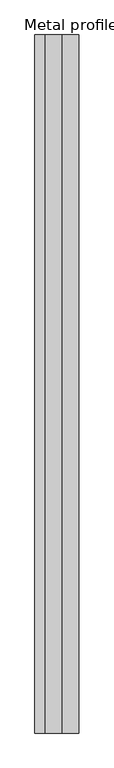
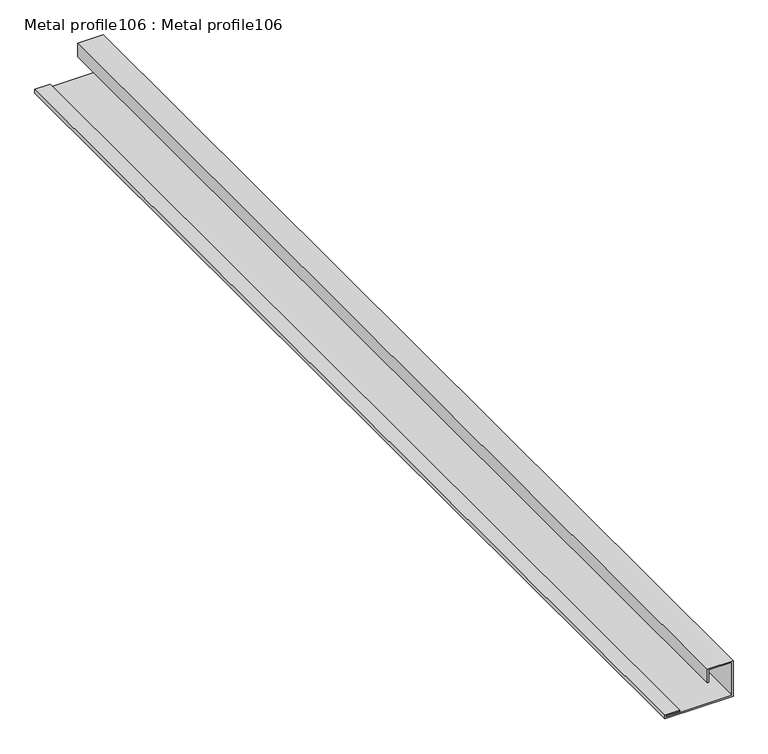
"""IFC4 building model written with IfcOpenShell, lengths in millimetres: proxy geometry, Metal profile106 : Metal profile106."""

from ifc_helpers import new_model, si_unit, frame, origin, place, context, project, spatial, polyline, outline, extrude, source, transform, mapped, element, save


def metal_profile106_metal_profile106_b8870bb5(model_context):
    return source(origin(), model_context, "Body", "SweptSolid", [
        extrude(outline(polyline([(41775.6266591, 6062.2987736), (41777.6266591, 6062.2987736), (41777.6266591, 6034.53559), (41770.7594716, 6034.53559), (41770.7594716, 6159.8011697), (41839.5329091, 6159.8011697), (41839.5329091, 6112.7894962), (41813.4391591, 6112.7894962), (41813.4391591, 6114.7894962), (41837.5329091, 6114.7894962), (41837.5329091, 6157.8011697), (41772.7594716, 6157.8011697), (41772.7594716, 6036.53559), (41775.6266591, 6036.53559), (41775.6266591, 6062.2987736)])), frame((0.0, 2217.3609988, 0.0), z_axis=(0.0, 1.0, 0.0), x_axis=(0.0, 0.0, 1.0)), (0.0, 0.0, 1.0), 2000.0),
    ])


if __name__ == "__main__":
    model = new_model("IFC4")
    model_context = context("Model", 3, world=origin())
    ifc_project = project(units=[si_unit("LENGTHUNIT", "METRE", prefix="MILLI")], contexts=[model_context])
    site = spatial("IfcSite", under=ifc_project)
    building = spatial("IfcBuilding", under=site)
    placement = place(None, origin())
    metal_profile106_metal_profile106_shape = metal_profile106_metal_profile106_b8870bb5(model_context)
    element("IfcBuildingElementProxy", 1, Name="Metal profile106 : Metal profile106", ObjectType="Metal profile106 : Metal profile106", at=placement, inside=building, context=model_context, shape_type="MappedRepresentation", body=[
        mapped(metal_profile106_metal_profile106_shape, transform((0.0, 0.0, 0.0), x_axis=(1.0, 0.0, 0.0), y_axis=(0.0, 1.0, 0.0), z_axis=(0.0, 0.0, 1.0))),
    ])
    save(model, "model.ifc")

# Revit data of these elements
# Type "Metal profile106 : Metal profile106"
#   NameOverride = "Metal profile106"
# Element 1 (IfcBuildingElementProxy, "Metal profile106 : Metal profile106")
#   Materials on its faces: "RECEIVER TRIM"
# Materials
#   "RECEIVER TRIM": class "Unassigned", colour RGB 245 226 176, transparency 0, Cost = 0
